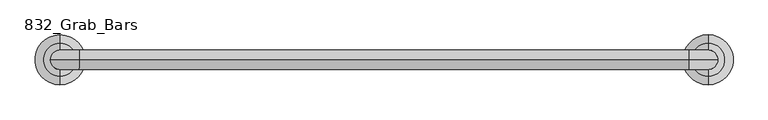
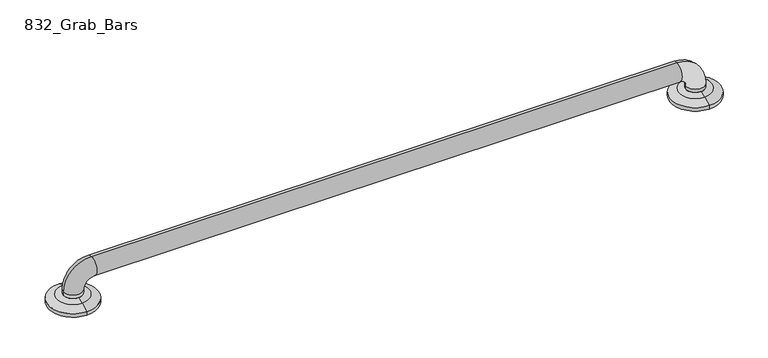
"""IFC4 building model written with IfcOpenShell, lengths in millimetres: proxy geometry, 832_Grab_Bars : 8320-001420."""

from ifc_helpers import new_model, si_unit, point, frame, origin, place, context, project, spatial, polyline, circle_curve, ellipse_curve, trimmed, source, transform, mapped, element, save
from ifc_brep_helpers import plane_surface, cylinder_surface, revolved_surface, advanced_brep


def proxy_832_grab_bars_8b3c1caf(model_context):
    return source(origin(), model_context, "Body", "AdvancedBrep", [
        advanced_brep(
        [(-439.7375, 564.1630987, 13.1934507), (-439.7375, 577.85, 6.35), (-439.7375, 495.3, 6.35), (-439.7375, 508.9869013, 13.1934507), (-439.7375, 520.3461266, 15.875), (-439.7375, 552.8038734, 15.875), (-439.7375, 520.7, 15.875), (-455.6125, 536.575, 15.875), (-439.7375, 552.45, 15.875), (-423.8625, 536.575, 15.875), (-439.7375, 577.85, 0.0), (-439.7375, 552.45, 0.0), (-439.7375, 536.575, 0.0), (-439.7375, 520.7, 0.0), (-439.7375, 495.3, 0.0), (627.0625, 564.2276895, 13.1934507), (627.0625, 577.9145908, 6.35), (627.0625, 495.3645908, 6.35), (627.0625, 509.0514921, 13.1934507), (627.0625, 520.4107174, 15.875), (627.0625, 552.8684641, 15.875), (627.0625, 520.7, 15.875), (611.1875, 536.575, 15.875), (627.0625, 552.45, 15.875), (642.9375, 536.575, 15.875), (627.0625, 577.9145908, 0.0), (627.0625, 552.45, 0.0), (627.0625, 536.6395908, 0.0), (627.0625, 520.7, 0.0), (627.0625, 495.3645908, 0.0), (-455.6125, 536.575, 22.225), (-423.8625, 536.575, 22.225), (-407.9875, 536.575, 38.1), (-407.9875, 536.575, 69.85), (595.3125, 536.575, 38.1), (595.3125, 536.575, 69.85), (611.1875, 536.575, 22.225), (642.9375, 536.575, 22.225)],
        [
            (0, 1),
            (1, 2, circle_curve(frame((-439.7375, 536.575, 6.35), z_axis=(0.0, 0.0, 1.0), x_axis=(0.0, -1.0, 0.0)), 41.275)),
            (2, 3),
            (3, 0, circle_curve(frame((-439.7375, 536.575, 13.1934507), z_axis=(0.0, 0.0, -1.0), x_axis=(0.0, -1.0, 0.0)), 27.5880987)),
            (2, 1, circle_curve(frame((-439.7375, 536.575, 6.35), z_axis=(0.0, 0.0, 1.0), x_axis=(0.0, -1.0, 0.0)), 41.275)),
            (0, 3, circle_curve(frame((-439.7375, 536.575, 13.1934507), z_axis=(0.0, 0.0, -1.0), x_axis=(0.0, -1.0, 0.0)), 27.5880987)),
            (3, 4, circle_curve(frame((-439.7375, 520.3461266, -9.525), z_axis=(-1.0, 0.0, 0.0), x_axis=(0.0, 0.0, -1.0)), 25.4)),
            (4, 5, circle_curve(frame((-439.7375, 536.575, 15.875), z_axis=(0.0, 0.0, -1.0), x_axis=(0.0, -1.0, 0.0)), 16.2288734)),
            (5, 0, circle_curve(frame((-439.7375, 552.8038734, -9.525), z_axis=(-1.0, 0.0, 0.0), x_axis=(0.0, 0.0, -1.0)), 25.4)),
            (5, 4, circle_curve(frame((-439.7375, 536.575, 15.875), z_axis=(0.0, 0.0, -1.0), x_axis=(0.0, -1.0, 0.0)), 16.2288734)),
            (4, 6),
            (6, 7, circle_curve(frame((-439.7375, 536.575, 15.875), z_axis=(0.0, 0.0, -1.0), x_axis=(1.0, 0.0, 0.0)), 15.875)),
            (7, 8, circle_curve(frame((-439.7375, 536.575, 15.875), z_axis=(0.0, 0.0, -1.0), x_axis=(1.0, 0.0, 0.0)), 15.875)),
            (8, 5),
            (8, 9, circle_curve(frame((-439.7375, 536.575, 15.875), z_axis=(0.0, 0.0, -1.0), x_axis=(1.0, 0.0, 0.0)), 15.875)),
            (9, 6, circle_curve(frame((-439.7375, 536.575, 15.875), z_axis=(0.0, 0.0, -1.0), x_axis=(1.0, 0.0, 0.0)), 15.875)),
            (10, 11),
            (11, 12),
            (12, 13),
            (13, 14),
            (14, 10, circle_curve(frame((-439.7375, 536.575, 0.0), z_axis=(0.0, 0.0, -1.0), x_axis=(0.0, -1.0, 0.0)), 41.275)),
            (10, 14, circle_curve(frame((-439.7375, 536.575, 0.0), z_axis=(0.0, 0.0, -1.0), x_axis=(0.0, -1.0, 0.0)), 41.275)),
            (1, 10),
            (14, 2),
            (15, 16),
            (16, 17, circle_curve(frame((627.0625, 536.6395908, 6.35), z_axis=(0.0, 0.0, 1.0), x_axis=(0.0, -1.0, 0.0)), 41.275)),
            (17, 18),
            (18, 15, circle_curve(frame((627.0625, 536.6395908, 13.1934507), z_axis=(0.0, 0.0, -1.0), x_axis=(0.0, -1.0, 0.0)), 27.5880987)),
            (17, 16, circle_curve(frame((627.0625, 536.6395908, 6.35), z_axis=(0.0, 0.0, 1.0), x_axis=(0.0, -1.0, 0.0)), 41.275)),
            (15, 18, circle_curve(frame((627.0625, 536.6395908, 13.1934507), z_axis=(0.0, 0.0, -1.0), x_axis=(0.0, -1.0, 0.0)), 27.5880987)),
            (18, 19, circle_curve(frame((627.0625, 520.4107174, -9.525), z_axis=(-1.0, 0.0, 0.0), x_axis=(0.0, 0.0, -1.0)), 25.4)),
            (19, 20, circle_curve(frame((627.0625, 536.6395908, 15.875), z_axis=(0.0, 0.0, -1.0), x_axis=(0.0, -1.0, 0.0)), 16.2288734)),
            (20, 15, circle_curve(frame((627.0625, 552.8684641, -9.525), z_axis=(-1.0, 0.0, 0.0), x_axis=(0.0, 0.0, -1.0)), 25.4)),
            (20, 19, circle_curve(frame((627.0625, 536.6395908, 15.875), z_axis=(0.0, 0.0, -1.0), x_axis=(0.0, -1.0, 0.0)), 16.2288734)),
            (19, 21),
            (21, 22, circle_curve(frame((627.0625, 536.575, 15.875), z_axis=(0.0, 0.0, -1.0), x_axis=(-1.0, 0.0, 0.0)), 15.875)),
            (22, 23, circle_curve(frame((627.0625, 536.575, 15.875), z_axis=(0.0, 0.0, -1.0), x_axis=(-1.0, 0.0, 0.0)), 15.875)),
            (23, 20),
            (23, 24, circle_curve(frame((627.0625, 536.575, 15.875), z_axis=(0.0, 0.0, -1.0), x_axis=(-1.0, 0.0, 0.0)), 15.875)),
            (24, 21, circle_curve(frame((627.0625, 536.575, 15.875), z_axis=(0.0, 0.0, -1.0), x_axis=(-1.0, 0.0, 0.0)), 15.875)),
            (25, 26),
            (26, 27),
            (27, 28),
            (28, 29),
            (29, 25, circle_curve(frame((627.0625, 536.6395908, 0.0), z_axis=(0.0, 0.0, -1.0), x_axis=(0.0, -1.0, 0.0)), 41.275)),
            (25, 29, circle_curve(frame((627.0625, 536.6395908, 0.0), z_axis=(0.0, 0.0, -1.0), x_axis=(0.0, -1.0, 0.0)), 41.275)),
            (16, 25),
            (29, 17),
            (30, 7),
            (9, 31),
            (31, 30, circle_curve(frame((-439.7375, 536.575, 22.225), z_axis=(0.0, 0.0, -1.0), x_axis=(1.0, 0.0, 0.0)), 15.875)),
            (30, 31, circle_curve(frame((-439.7375, 536.575, 22.225), z_axis=(0.0, 0.0, -1.0), x_axis=(1.0, 0.0, 0.0)), 15.875)),
            (31, 32, circle_curve(frame((-407.9875, 536.575, 22.225), z_axis=(0.0, 1.0, 0.0), x_axis=(-1.0, 0.0, 0.0)), 15.875)),
            (32, 33, circle_curve(frame((-407.9875, 536.575, 53.975), z_axis=(-1.0, 0.0, 0.0), x_axis=(0.0, 0.0, -1.0)), 15.875)),
            (33, 30, circle_curve(frame((-407.9875, 536.575, 22.225), z_axis=(0.0, -1.0, 0.0), x_axis=(-1.0, 0.0, 0.0)), 47.625)),
            (33, 32, circle_curve(frame((-407.9875, 536.575, 53.975), z_axis=(-1.0, 0.0, 0.0), x_axis=(0.0, 0.0, -1.0)), 15.875)),
            (32, 34),
            (34, 35, circle_curve(frame((595.3125, 536.575, 53.975), z_axis=(-1.0, 0.0, 0.0), x_axis=(0.0, 0.0, -1.0)), 15.875)),
            (35, 33),
            (35, 34, circle_curve(frame((595.3125, 536.575, 53.975), z_axis=(-1.0, 0.0, 0.0), x_axis=(0.0, 0.0, -1.0)), 15.875)),
            (34, 36, circle_curve(frame((595.3125, 536.575, 22.225), z_axis=(0.0, 1.0, 0.0), x_axis=(0.0, 0.0, 1.0)), 15.875)),
            (36, 37, circle_curve(frame((627.0625, 536.575, 22.225), z_axis=(0.0, 0.0, 1.0), x_axis=(-1.0, 0.0, 0.0)), 15.875)),
            (37, 35, circle_curve(frame((595.3125, 536.575, 22.225), z_axis=(0.0, -1.0, 0.0), x_axis=(0.0, 0.0, 1.0)), 47.625)),
            (37, 36, circle_curve(frame((627.0625, 536.575, 22.225), z_axis=(0.0, 0.0, 1.0), x_axis=(-1.0, 0.0, 0.0)), 15.875)),
            (36, 22),
            (24, 37),
        ],
        [
            revolved_surface(polyline([(-439.7375, 495.3, 6.35), (-439.7375, 508.9869013, 13.1934507)]), (-439.7375, 536.575, 31.75), (0.0, 0.0, 1.0)),
            revolved_surface(trimmed(ellipse_curve(frame((-439.7375, 520.3461266, -9.525), z_axis=(-1.0, 0.0, 0.0), x_axis=(0.0, 0.0, -1.0)), 25.4, 25.4), [point((-439.7375, 508.9869013, 13.1934507))], [point((-439.7375, 520.3461266, 15.875))], True, "CARTESIAN"), (-439.7375, 536.575, 31.75), (0.0, 0.0, 1.0)),
            plane_surface(frame((-439.7375, 536.575, 15.875), z_axis=(0.0, 0.0, 1.0), x_axis=(0.0, -1.0, 0.0))),
            plane_surface(frame((-439.7375, 536.575, 0.0), z_axis=(0.0, 0.0, -1.0), x_axis=(0.0, -1.0, 0.0))),
            cylinder_surface(frame((-439.7375, 536.575, 31.75), z_axis=(0.0, 0.0, 1.0), x_axis=(0.0, -1.0, 0.0)), 41.275),
            revolved_surface(polyline([(627.0625, 495.3645908, 6.35), (627.0625, 509.0514921, 13.1934507)]), (627.0625, 536.6395908, 31.75), (0.0, 0.0, 1.0)),
            revolved_surface(trimmed(ellipse_curve(frame((627.0625, 520.4107174, -9.525), z_axis=(-1.0, 0.0, 0.0), x_axis=(0.0, 0.0, -1.0)), 25.4, 25.4), [point((627.0625, 509.0514921, 13.1934507))], [point((627.0625, 520.4107174, 15.875))], True, "CARTESIAN"), (627.0625, 536.6395908, 31.75), (0.0, 0.0, 1.0)),
            plane_surface(frame((627.0625, 536.6395908, 15.875), z_axis=(0.0, 0.0, 1.0), x_axis=(0.0, -1.0, 0.0))),
            plane_surface(frame((627.0625, 536.6395908, 0.0), z_axis=(0.0, 0.0, -1.0), x_axis=(0.0, -1.0, 0.0))),
            cylinder_surface(frame((627.0625, 536.6395908, 31.75), z_axis=(0.0, 0.0, 1.0), x_axis=(0.0, -1.0, 0.0)), 41.275),
            cylinder_surface(frame((-439.7375, 536.575, 0.0), z_axis=(0.0, 0.0, -1.0), x_axis=(1.0, 0.0, 0.0)), 15.875),
            revolved_surface(trimmed(ellipse_curve(frame((-439.7375, 536.575, 22.225), z_axis=(0.0, 0.0, 1.0), x_axis=(1.0, 0.0, 0.0)), 15.875, 15.875), [point((-455.6125, 536.575, 22.225))], [point((-423.8625, 536.575, 22.225))], True, "CARTESIAN"), (-407.9875, 536.575, 22.225), (0.0, -1.0, 0.0)),
            revolved_surface(trimmed(ellipse_curve(frame((-439.7375, 536.575, 22.225), z_axis=(0.0, 0.0, 1.0), x_axis=(1.0, 0.0, 0.0)), 15.875, 15.875), [point((-423.8625, 536.575, 22.225))], [point((-455.6125, 536.575, 22.225))], True, "CARTESIAN"), (-407.9875, 536.575, 22.225), (0.0, -1.0, 0.0)),
            cylinder_surface(frame((-407.9875, 536.575, 53.975), z_axis=(-1.0, 0.0, 0.0), x_axis=(0.0, 0.0, -1.0)), 15.875),
            revolved_surface(trimmed(ellipse_curve(frame((595.3125, 536.575, 53.975), z_axis=(1.0, 0.0, 0.0), x_axis=(0.0, 0.0, -1.0)), 15.875, 15.875), [point((595.3125, 536.575, 69.85))], [point((595.3125, 536.575, 38.1))], True, "CARTESIAN"), (595.3125, 536.575, 22.225), (0.0, -1.0, 0.0)),
            revolved_surface(trimmed(ellipse_curve(frame((595.3125, 536.575, 53.975), z_axis=(1.0, 0.0, 0.0), x_axis=(0.0, 0.0, -1.0)), 15.875, 15.875), [point((595.3125, 536.575, 38.1))], [point((595.3125, 536.575, 69.85))], True, "CARTESIAN"), (595.3125, 536.575, 22.225), (0.0, -1.0, 0.0)),
            cylinder_surface(frame((627.0625, 536.575, 22.225), z_axis=(0.0, 0.0, 1.0), x_axis=(-1.0, 0.0, 0.0)), 15.875),
        ],
        [
            (0, [[1, 2, 3, 4]]),
            (0, [[5, -1, 6, -3]]),
            (1, [[7, 8, 9, -4]]),
            (1, [[-9, 10, -7, -6]]),
            (2, [[11, 12, 13, 14, -8]]),
            (2, [[-14, 15, 16, -11, -10]]),
            (3, [[17, 18, 19, 20, 21]]),
            (3, [[-20, -19, -18, -17, 22]]),
            (4, [[23, -21, 24, -2]]),
            (4, [[-24, -22, -23, -5]]),
            (5, [[25, 26, 27, 28]]),
            (5, [[29, -25, 30, -27]]),
            (6, [[31, 32, 33, -28]]),
            (6, [[-33, 34, -31, -30]]),
            (7, [[35, 36, 37, 38, -32]]),
            (7, [[-38, 39, 40, -35, -34]]),
            (8, [[41, 42, 43, 44, 45]]),
            (8, [[-44, -43, -42, -41, 46]]),
            (9, [[47, -45, 48, -26]]),
            (9, [[-48, -46, -47, -29]]),
            (10, [[49, -12, -16, 50, 51]]),
            (10, [[-50, -15, -13, -49, 52]]),
            (11, [[53, 54, 55, -51]]),
            (12, [[-55, 56, -53, -52]]),
            (13, [[57, 58, 59, -54]]),
            (13, [[-59, 60, -57, -56]]),
            (14, [[61, 62, 63, -58]]),
            (15, [[-63, 64, -61, -60]]),
            (16, [[65, -36, -40, 66, -62]]),
            (16, [[-66, -39, -37, -65, -64]]),
        ],
    ),
    ])


if __name__ == "__main__":
    model = new_model("IFC4")
    model_context = context("Model", 3, world=origin())
    ifc_project = project(units=[si_unit("LENGTHUNIT", "METRE", prefix="MILLI")], contexts=[model_context])
    site = spatial("IfcSite", under=ifc_project)
    building = spatial("IfcBuilding", under=site)
    placement = place(None, origin())
    proxy_832_grab_bars_shape = proxy_832_grab_bars_8b3c1caf(model_context)
    element("IfcBuildingElementProxy", 1, Name="832_Grab_Bars : 8320-001420", ObjectType="832_Grab_Bars : 8320-001420", at=placement, inside=building, context=model_context, shape_type="MappedRepresentation", body=[
        mapped(proxy_832_grab_bars_shape, transform((0.0, 0.0, 0.0), x_axis=(1.0, 0.0, 0.0), y_axis=(0.0, 1.0, 0.0), z_axis=(0.0, 0.0, 1.0))),
    ])
    save(model, "model.ifc")

# Revit data of these elements
# Type "832_Grab_Bars : 8320-001420"
#   Warranty Information = "Complete unit, one (1) year"
#   Version = "1.0"
#   Technical Data = "http://www.bradleycorp.com/products/techdata/8820.pdf"
#   URL = "www.bradleycorp.com"
#   Type Comments = "All grab bar configurations are specified using centerline to centerline dimensions."
#   OmniClass Title = ""
#   Modeling Code = ""
#   Model = "8320-001420"
#   Material Note = "FLANGES - 13GA., ESCUTCHEONS - 22GA., TUBING - 18GA."
#   MasterFormat Section Title = ""
#   Manufacturer = "Bradley Corporation"
#   LEED Credit = ""
#   Instructions [instance default] = "This is a face mounted fixture."
#   Industry Standards = "ANSI Standard A117.1, ADA, ABA, ADAAG, UFAS"
#   Fire Rating = "None"
#   Description = "Grab Bars"
#   Copyright = "This Model Data is Property of Bradley Corporation"
#   Complies to NAFTA = "Yes"
#   Complies To Buy American Act = "Yes"
#   Assembly Code = "C1030200"
#   ADA Compliant = "Yes"
#   Radius = 15.875 mm
#   Percentage of Recycled Content = 64.98
#   Overall Length = 1149.35 mm
#   OmniClass Code = 0
#   MasterFormat Section Number = 0
#   Length = 1066.8 mm
#   Diameter = 31.75 mm
#   Default Elevation = 838.2 mm
#   Material and Finish = Bradley Corp Stainless Steel - Satin
# Element 1 (IfcBuildingElementProxy, "832_Grab_Bars : 8320-001420")
#   Materials on its faces: "Bradley Corp Stainless Steel - Satin"
# Materials
#   "Bradley Corp Stainless Steel - Satin": class "Metal", colour RGB 189 187 185, transparency 0, Manufacturer = "Bradley Corporation", URL = "www.bradleycorp.com", Description = "Stainless Steel - Satin Finish", Cost = 0
